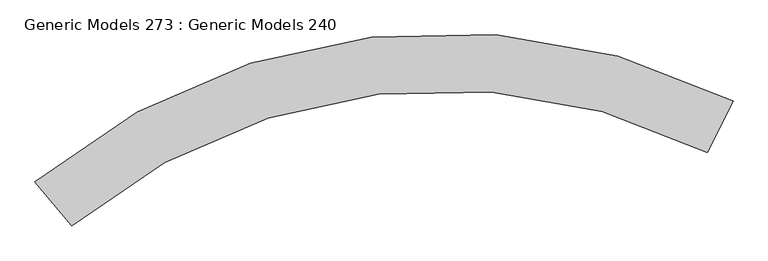
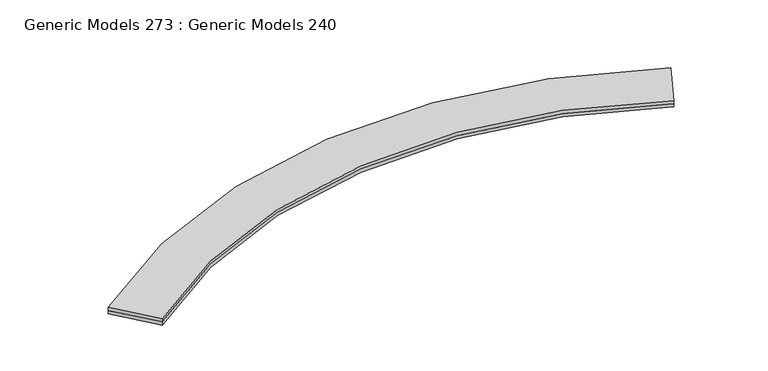
"""IFC4 building model written with IfcOpenShell, lengths in millimetres: proxy geometry, Generic Models 273 : Generic Models 240."""

from ifc_helpers import new_model, si_unit, point, frame, frame_2d, origin, place, context, project, spatial, polyline, circle_curve, trimmed, segment, composite_curve, outline, extrude, source, transform, mapped, element, save


def generic_models_273_generic_models_240_9af6f6b6(model_context):
    return source(origin(), model_context, "Body", "SweptSolid", [
        extrude(outline(composite_curve([segment(trimmed(circle_curve(frame_2d((-832.04683, -25139.2753781)), 3107.2218919), [point((-2826.380524, -22756.53305))], [point((562.7602224, -22362.7053408))], False, "CARTESIAN"), True, "CONTINUOUS"), segment(polyline([(562.7602224, -22362.7053408), (437.3397973, -22612.3732742)]), True, "CONTINUOUS"), segment(trimmed(circle_curve(frame_2d((-832.04683, -25139.2753781)), 2827.8218919), [point((437.3397973, -22612.3732742))], [point((-2647.050932, -22970.7881723))], True, "CARTESIAN"), True, "CONTINUOUS"), segment(polyline([(-2647.050932, -22970.7881723), (-2826.380524, -22756.53305)]), True, "CONTINUOUS")], self_intersect=False)), frame((0.0, 0.0, 1035.05), z_axis=(0.0, 0.0, 1.0), x_axis=(1.0, 0.0, 0.0)), (0.0, 0.0, 1.0), 19.05),
        extrude(outline(composite_curve([segment(trimmed(circle_curve(frame_2d((-832.04683, -25139.2753781)), 3107.2218919), [point((-2826.380524, -22756.53305))], [point((562.7602224, -22362.7053408))], False, "CARTESIAN"), True, "CONTINUOUS"), segment(polyline([(562.7602224, -22362.7053408), (437.3397973, -22612.3732742)]), True, "CONTINUOUS"), segment(trimmed(circle_curve(frame_2d((-832.04683, -25139.2753781)), 2827.8218919), [point((437.3397973, -22612.3732742))], [point((-2647.050932, -22970.7881723))], True, "CARTESIAN"), True, "CONTINUOUS"), segment(polyline([(-2647.050932, -22970.7881723), (-2826.380524, -22756.53305)]), True, "CONTINUOUS")], self_intersect=False)), frame((0.0, 0.0, 1054.1), z_axis=(0.0, 0.0, 1.0), x_axis=(1.0, 0.0, 0.0)), (0.0, 0.0, 1.0), 19.05),
    ])


if __name__ == "__main__":
    model = new_model("IFC4")
    model_context = context("Model", 3, world=origin())
    ifc_project = project(units=[si_unit("LENGTHUNIT", "METRE", prefix="MILLI")], contexts=[model_context])
    site = spatial("IfcSite", under=ifc_project)
    building = spatial("IfcBuilding", under=site)
    placement = place(None, origin())
    generic_models_273_generic_models_240_shape = generic_models_273_generic_models_240_9af6f6b6(model_context)
    element("IfcBuildingElementProxy", 1, Name="Generic Models 273 : Generic Models 240", ObjectType="Generic Models 273 : Generic Models 240", at=placement, inside=building, context=model_context, shape_type="MappedRepresentation", body=[
        mapped(generic_models_273_generic_models_240_shape, transform((0.0, 0.0, 0.0), x_axis=(1.0, 0.0, 0.0), y_axis=(0.0, 1.0, 0.0), z_axis=(0.0, 0.0, 1.0))),
    ])
    save(model, "model.ifc")

# Revit data of these elements
# Element 1 (IfcBuildingElementProxy, "Generic Models 273 : Generic Models 240")
#   Materials on its faces: "3/4\" PLYWOOD ,GRADE B FINISH (2x)"
# Materials
#   "3/4\" PLYWOOD ,GRADE B FINISH (2x)": class "Wood", colour RGB 48 37 22, transparency 0, Description = "Plywood, sheathing grade", Cost = 0
